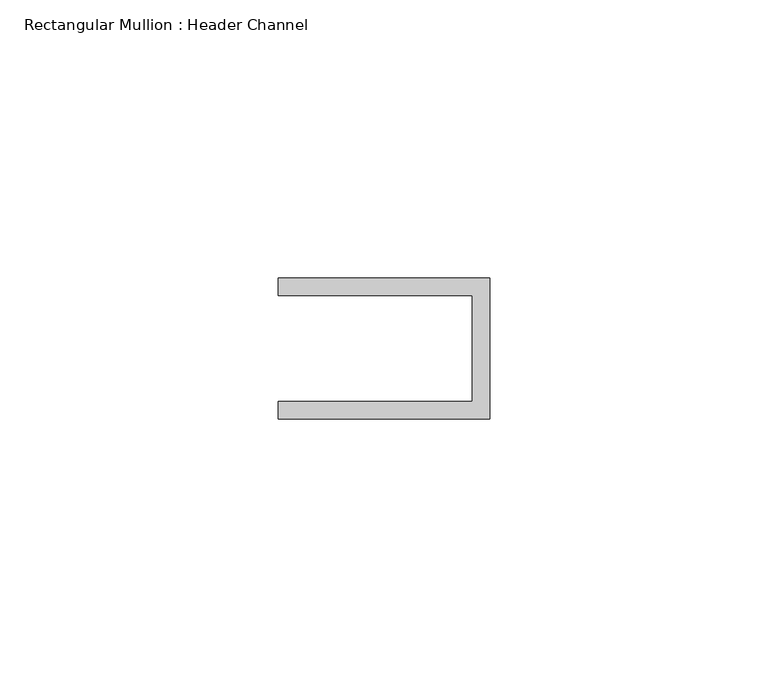
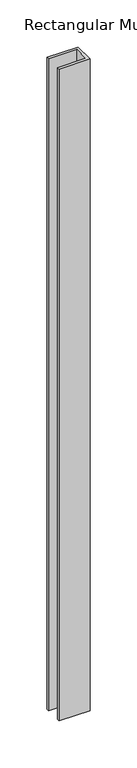
"""IFC4 building model written with IfcOpenShell, lengths in millimetres: member geometry, Rectangular Mullion : Header Channel."""

from ifc_helpers import new_model, si_unit, frame, origin, place, context, project, spatial, polyline, outline, extrude, source, transform, mapped, element, save


def rectangular_mullion_header_channel_b79a45dd(model_context):
    return source(origin(), model_context, "Body", "SweptSolid", [
        extrude(outline(polyline([(0.0, -12.7), (-38.1, -12.7), (-38.1, -9.525), (-3.175, -9.525), (-3.175, 9.525), (-38.1, 9.525), (-38.1, 12.7), (0.0, 12.7), (0.0, -12.7)])), frame((0.0, 0.0, -845.4185495), z_axis=(0.0, 0.0, 1.0), x_axis=(1.0, 0.0, 0.0)), (0.0, 0.0, 1.0), 845.4185495),
    ])


if __name__ == "__main__":
    model = new_model("IFC4")
    model_context = context("Model", 3, world=origin())
    ifc_project = project(units=[si_unit("LENGTHUNIT", "METRE", prefix="MILLI")], contexts=[model_context])
    site = spatial("IfcSite", under=ifc_project)
    building = spatial("IfcBuilding", under=site)
    placement = place(None, origin())
    rectangular_mullion_header_channel_shape = rectangular_mullion_header_channel_b79a45dd(model_context)
    element("IfcMember", 1, ObjectType="Rectangular Mullion : Header Channel", at=placement, inside=building, context=model_context, shape_type="MappedRepresentation", body=[
        mapped(rectangular_mullion_header_channel_shape, transform((0.0, 0.0, 0.0), x_axis=(1.0, 0.0, 0.0), y_axis=(0.0, 1.0, 0.0), z_axis=(0.0, 0.0, 1.0))),
    ])
    save(model, "model.ifc")

# Revit data of these elements
# Type "Rectangular Mullion : Header Channel"
#   built-in parameter 1007322 = 0.0833333 (stored number, unit not read)
#   built-in parameter 1007321 = -0.03125 (stored number, unit not read)
#   built-in parameter 1007320 = 0.0416667 (stored number, unit not read)
# Element 1 (IfcMember, "Rectangular Mullion : Header Channel")
#   Materials on its faces: "ALUM"
# Materials
#   "ALUM": class "Generic", colour RGB 157 157 157, transparency 0, Cost = 0
